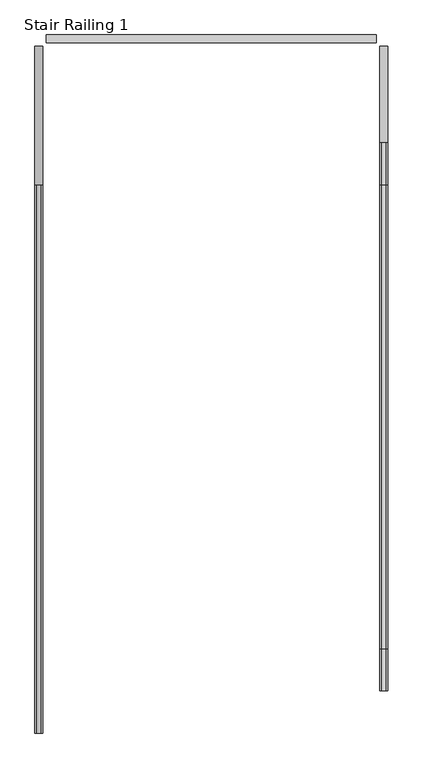
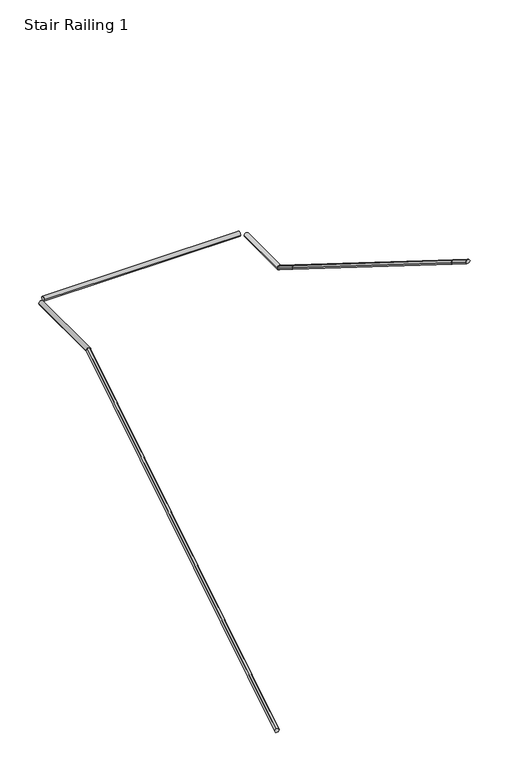
"""IFC4 building model written with IfcOpenShell, lengths in millimetres: railing geometry, Stair Railing 1."""

from ifc_helpers import new_model, si_unit, frame, origin, place, context, project, spatial, circle_curve, faceted_brep, source, transform, mapped, element, save
from ifc_brep_helpers import plane_surface, cylinder_surface, advanced_brep


def stair_railing_1_835fd4d1(model_context):
    return source(origin(), model_context, "Body", "SolidModel", [
        faceted_brep([(-2482.1134126, 56357.2066802, 9028.2888889), (-2469.4134126, 56357.2066802, 9050.2859341), (-2444.0134126, 56357.2066802, 9050.2859341), (-2431.3134126, 56357.2066802, 9028.2888889), (-2444.0134126, 56357.2066802, 9006.2918436), (-2469.4134126, 56357.2066802, 9006.2918436), (-2482.1134126, 52725.0066802, 6753.5777778), (-2469.4134126, 52725.0066802, 6731.5807325), (-2444.0134126, 52725.0066802, 6731.5807325), (-2431.3134126, 52725.0066802, 6753.5777778), (-2444.0134126, 52725.0066802, 6775.574823), (-2469.4134126, 52725.0066802, 6775.574823)], [[[0, 1, 2, 3, 4, 5]], [[6, 7, 8, 9, 10, 11]], [[1, 0, 6, 11]], [[2, 1, 11, 10]], [[3, 2, 10, 9]], [[4, 3, 9, 8]], [[5, 4, 8, 7]], [[0, 5, 7, 6]]]),
        advanced_brep(
        [(-2482.1134126, 57271.6066802, 9028.2888889), (-2431.3134126, 57271.6066802, 9028.2888889), (-2482.1134126, 56357.2066802, 9028.2888889), (-2431.3134126, 56357.2066802, 9028.2888889)],
        [
            (0, 1, circle_curve(frame((-2456.7134126, 57271.6066802, 9028.2888889), z_axis=(0.0, 1.0, 0.0), x_axis=(-0.9999999999999999, 0.0, 0.0)), 25.4)),
            (1, 0, circle_curve(frame((-2456.7134126, 57271.6066802, 9028.2888889), z_axis=(0.0, 1.0, 0.0), x_axis=(-0.9999999999999999, 0.0, 0.0)), 25.4)),
            (2, 3, circle_curve(frame((-2456.7134126, 56357.2066802, 9028.2888889), z_axis=(0.0, -1.0, 0.0), x_axis=(-0.9999999999999999, 0.0, 0.0)), 25.4)),
            (3, 2, circle_curve(frame((-2456.7134126, 56357.2066802, 9028.2888889), z_axis=(0.0, -1.0, 0.0), x_axis=(-0.9999999999999999, 0.0, 0.0)), 25.4)),
            (0, 2),
            (3, 1),
        ],
        [
            plane_surface(frame((-2482.1134126, 57271.6066802, 9002.8888889), z_axis=(0.0, 1.0, 0.0), x_axis=(0.0, 0.0, 1.0))),
            plane_surface(frame((-2482.1134126, 56357.2066802, 9002.8888889), z_axis=(0.0, -1.0, 0.0), x_axis=(0.0, 0.0, -1.0))),
            cylinder_surface(frame((-2456.7134126, 56357.2066802, 9028.2888889), z_axis=(0.0, 0.9999999999999999, 0.0), x_axis=(-0.9999999999999999, 0.0, 0.0)), 25.4),
        ],
        [
            (0, [[1, 2]]),
            (1, [[3, 4]]),
            (2, [[-1, 5, -4, 6]]),
            (2, [[-2, -6, -3, -5]]),
        ],
    ),
        advanced_brep(
        [(-222.5891104, 57347.8066802, 9028.2888889), (-222.5891104, 57297.0066802, 9028.2888889), (-2405.9134126, 57347.8066802, 9028.2888889), (-2405.9134126, 57297.0066802, 9028.2888889)],
        [
            (0, 1, circle_curve(frame((-222.5891104, 57322.4066802, 9028.2888889), z_axis=(1.0, 0.0, 0.0), x_axis=(0.0, 1.0, 0.0)), 25.4)),
            (1, 0, circle_curve(frame((-222.5891104, 57322.4066802, 9028.2888889), z_axis=(1.0, 0.0, 0.0), x_axis=(0.0, 1.0, 0.0)), 25.4)),
            (2, 3, circle_curve(frame((-2405.9134126, 57322.4066802, 9028.2888889), z_axis=(-1.0, 0.0, 0.0), x_axis=(0.0, 1.0, 0.0)), 25.4)),
            (3, 2, circle_curve(frame((-2405.9134126, 57322.4066802, 9028.2888889), z_axis=(-1.0, 0.0, 0.0), x_axis=(0.0, 1.0, 0.0)), 25.4)),
            (0, 2),
            (3, 1),
        ],
        [
            plane_surface(frame((-222.5891104, 57347.8066802, 9002.8888889), z_axis=(1.0, 0.0, 0.0), x_axis=(0.0, 1.0, 0.0))),
            plane_surface(frame((-2405.9134126, 57347.8066802, 9002.8888889), z_axis=(-1.0, 0.0, 0.0), x_axis=(0.0, -1.0, 0.0))),
            cylinder_surface(frame((-2405.9134126, 57322.4066802, 9028.2888889), z_axis=(1.0, 0.0, 0.0), x_axis=(0.0, 1.0, 0.0)), 25.4),
        ],
        [
            (0, [[1, 2]]),
            (1, [[3, 4]]),
            (2, [[-1, 5, -4, 6]]),
            (2, [[-2, -6, -3, -5]]),
        ],
    ),
        advanced_brep(
        [(-146.3891104, 56636.6066802, 9028.2888889), (-197.1891104, 56636.6066802, 9028.2888889), (-146.3891104, 57271.6066802, 9028.2888889), (-197.1891104, 57271.6066802, 9028.2888889)],
        [
            (0, 1, circle_curve(frame((-171.7891104, 56636.6066802, 9028.2888889), z_axis=(0.0, -1.0, 0.0), x_axis=(1.0, 0.0, 0.0)), 25.4)),
            (1, 0, circle_curve(frame((-171.7891104, 56636.6066802, 9028.2888889), z_axis=(0.0, -1.0, 0.0), x_axis=(1.0, 0.0, 0.0)), 25.4)),
            (2, 3, circle_curve(frame((-171.7891104, 57271.6066802, 9028.2888889), z_axis=(0.0, 1.0, 0.0), x_axis=(1.0, 0.0, 0.0)), 25.4)),
            (3, 2, circle_curve(frame((-171.7891104, 57271.6066802, 9028.2888889), z_axis=(0.0, 1.0, 0.0), x_axis=(1.0, 0.0, 0.0)), 25.4)),
            (0, 2),
            (3, 1),
        ],
        [
            plane_surface(frame((-146.3891104, 56636.6066802, 9002.8888889), z_axis=(0.0, -1.0, 0.0), x_axis=(0.0, 0.0, -1.0))),
            plane_surface(frame((-146.3891104, 57271.6066802, 9002.8888889), z_axis=(0.0, 1.0, 0.0), x_axis=(0.0, 0.0, 1.0))),
            cylinder_surface(frame((-171.7891104, 57271.6066802, 9028.2888889), z_axis=(0.0, -1.0, 0.0), x_axis=(1.0, 0.0, 0.0)), 25.4),
        ],
        [
            (0, [[1, 2]]),
            (1, [[3, 4]]),
            (2, [[-1, 5, -4, 6]]),
            (2, [[-2, -6, -3, -5]]),
        ],
    ),
        faceted_brep([(-146.3891104, 56357.2066802, 9203.2666667), (-159.0891104, 56357.2066802, 9225.2637119), (-184.4891104, 56357.2066802, 9225.2637119), (-197.1891104, 56357.2066802, 9203.2666667), (-184.4891104, 56357.2066802, 9181.2696214), (-159.0891104, 56357.2066802, 9181.2696214), (-146.3891104, 56636.6066802, 9028.2888889), (-159.0891104, 56636.6066802, 9006.2918436), (-184.4891104, 56636.6066802, 9006.2918436), (-197.1891104, 56636.6066802, 9028.2888889), (-184.4891104, 56636.6066802, 9050.2859341), (-159.0891104, 56636.6066802, 9050.2859341)], [[[0, 1, 2, 3, 4, 5]], [[6, 7, 8, 9, 10, 11]], [[1, 0, 6, 11]], [[2, 1, 11, 10]], [[3, 2, 10, 9]], [[4, 3, 9, 8]], [[5, 4, 8, 7]], [[0, 5, 7, 6]]]),
        faceted_brep([(-146.3891104, 53283.8066802, 11128.0222222), (-159.0891104, 53283.8066802, 11150.0192675), (-184.4891104, 53283.8066802, 11150.0192675), (-197.1891104, 53283.8066802, 11128.0222222), (-184.4891104, 53283.8066802, 11106.025177), (-159.0891104, 53283.8066802, 11106.025177), (-146.3891104, 56357.2066802, 9203.2666667), (-159.0891104, 56357.2066802, 9181.2696214), (-184.4891104, 56357.2066802, 9181.2696214), (-197.1891104, 56357.2066802, 9203.2666667), (-184.4891104, 56357.2066802, 9225.2637119), (-159.0891104, 56357.2066802, 9225.2637119)], [[[0, 1, 2, 3, 4, 5]], [[6, 7, 8, 9, 10, 11]], [[1, 0, 6, 11]], [[2, 1, 11, 10]], [[3, 2, 10, 9]], [[4, 3, 9, 8]], [[5, 4, 8, 7]], [[0, 5, 7, 6]]]),
        faceted_brep([(-146.3891104, 53004.4066802, 11303.0), (-159.0891104, 53004.4066802, 11324.9970453), (-184.4891104, 53004.4066802, 11324.9970453), (-197.1891104, 53004.4066802, 11303.0), (-184.4891104, 53004.4066802, 11281.0029547), (-159.0891104, 53004.4066802, 11281.0029547), (-146.3891104, 53283.8066802, 11128.0222222), (-159.0891104, 53283.8066802, 11106.025177), (-184.4891104, 53283.8066802, 11106.025177), (-197.1891104, 53283.8066802, 11128.0222222), (-184.4891104, 53283.8066802, 11150.0192675), (-159.0891104, 53283.8066802, 11150.0192675)], [[[0, 1, 2, 3, 4, 5]], [[6, 7, 8, 9, 10, 11]], [[1, 0, 6, 11]], [[2, 1, 11, 10]], [[3, 2, 10, 9]], [[4, 3, 9, 8]], [[5, 4, 8, 7]], [[0, 5, 7, 6]]]),
    ])


if __name__ == "__main__":
    model = new_model("IFC4")
    model_context = context("Model", 3, world=origin())
    ifc_project = project(units=[si_unit("LENGTHUNIT", "METRE", prefix="MILLI")], contexts=[model_context])
    site = spatial("IfcSite", under=ifc_project)
    building = spatial("IfcBuilding", under=site)
    placement = place(None, origin())
    stair_railing_1_shape = stair_railing_1_835fd4d1(model_context)
    element("IfcRailing", 1, ObjectType="Stair Railing 1", at=placement, inside=building, context=model_context, shape_type="MappedRepresentation", body=[
        mapped(stair_railing_1_shape, transform((0.0, 0.0, 0.0), x_axis=(1.0, 0.0, 0.0), y_axis=(0.0, 1.0, 0.0), z_axis=(0.0, 0.0, 1.0))),
    ])
    save(model, "model.ifc")
